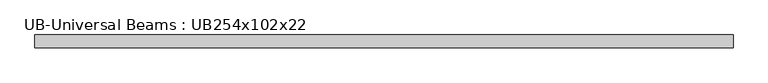
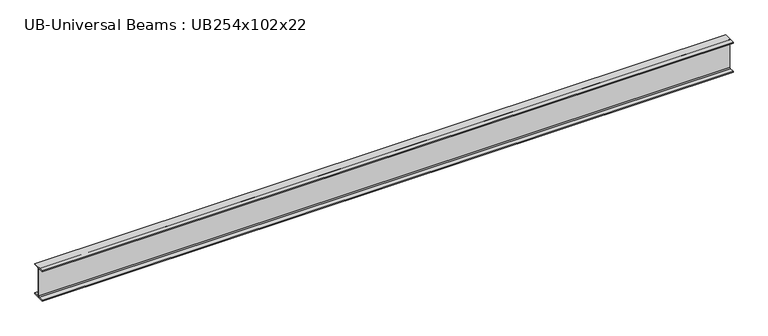
"""IFC4 building model written with IfcOpenShell, lengths in millimetres: beam geometry, UB-Universal Beams : UB254x102x22."""

import ifcopenshell
import ifcopenshell.guid

model = None  # the IFC model being written
_history = None  # IfcOwnerHistory: only IFC2X3 demands one
_inside = {}  # id of a spatial element -> (the spatial element, [elements in it])
_under = {}  # id of a project, library or spatial element -> (it, [spatial elements below it])
_declared = {}  # id of a project -> (the project, [libraries it declares])
_typed = {}  # id of a type object -> (the type object, [elements of that type])
_made_of = {}  # id of a material, layer set ... -> (it, [elements and type objects made of it])


def new_model(schema):
    """Start an empty IFC model of exactly this schema.

    Asked for "IFC4X3", IfcOpenShell would pick the latest addendum, in which some entities
    have other attributes; the version numbers below select the first issue.
    IFC2X3 requires an IfcOwnerHistory on every rooted entity: one is made here for all.
    """
    global model, _history
    if schema == "IFC4X3":
        model = ifcopenshell.file(schema_version=(4, 3, 0, 0))
    else:
        model = ifcopenshell.file(schema=schema)
    _inside.clear()
    _under.clear()
    _declared.clear()
    _typed.clear()
    _made_of.clear()
    _history = None
    if model.schema == "IFC2X3":
        org = make("IfcOrganization", Name="unknown")
        user = make(
            "IfcPersonAndOrganization",
            ThePerson=make("IfcPerson", FamilyName="unknown"),
            TheOrganization=org,
        )
        app = make(
            "IfcApplication",
            ApplicationDeveloper=org,
            Version="unknown",
            ApplicationFullName="unknown",
            ApplicationIdentifier="unknown",
        )
        _history = make(
            "IfcOwnerHistory",
            OwningUser=user,
            OwningApplication=app,
            ChangeAction="ADDED",
            CreationDate=0,
        )
    return model


def make(cls, **values):
    """One entity of the class cls with the attributes given. An attribute that is None is left unset."""
    return model.create_entity(
        cls, **{name: value for name, value in values.items() if value is not None}
    )


def rooted(cls, **values):
    """An entity with a GlobalId (a new one), such as an element, a storey or a relation."""
    return make(cls, GlobalId=ifcopenshell.guid.new(), OwnerHistory=_history, **values)


def si_unit(unit_type, name, prefix=None):
    """IfcSIUnit, for example si_unit("LENGTHUNIT", "METRE", prefix="MILLI")."""
    return make("IfcSIUnit", UnitType=unit_type, Prefix=prefix, Name=name)


def assignment(units):
    """IfcUnitAssignment: the units of a project."""
    return None if units is None else make("IfcUnitAssignment", Units=units)


def point(xyz):
    """IfcCartesianPoint."""
    return None if xyz is None else make("IfcCartesianPoint", Coordinates=xyz)


def direction(xyz):
    """IfcDirection."""
    return None if xyz is None else make("IfcDirection", DirectionRatios=xyz)


def frame(location, z_axis=None, x_axis=None):
    """IfcAxis2Placement3D, a coordinate frame: its origin and axes. An axis left out is left unset."""
    return make(
        "IfcAxis2Placement3D",
        Location=point(location),
        Axis=direction(z_axis),
        RefDirection=direction(x_axis),
    )


def frame_2d(location, x_axis=None):
    """IfcAxis2Placement2D, a coordinate frame in the plane: its origin and x axis."""
    return make(
        "IfcAxis2Placement2D", Location=point(location), RefDirection=direction(x_axis)
    )


def origin():
    """The frame at (0, 0, 0) with its axes left unset."""
    return frame((0.0, 0.0, 0.0))


def place(relative_to, where):
    """IfcLocalPlacement: puts the frame where relative to a parent placement (None: the world)."""
    return make(
        "IfcLocalPlacement", PlacementRelTo=relative_to, RelativePlacement=where
    )


def context(
    kind, dimensions, precision=None, world=None, true_north=None, identifier=None
):
    """IfcGeometricRepresentationContext, for example the 3D "Model" context."""
    return make(
        "IfcGeometricRepresentationContext",
        ContextIdentifier=identifier,
        ContextType=kind,
        CoordinateSpaceDimension=dimensions,
        Precision=precision,
        WorldCoordinateSystem=world,
        TrueNorth=true_north,
    )


def project(units=None, contexts=None):
    """IfcProject with its units and contexts."""
    return rooted(
        "IfcProject",
        Name="project",
        RepresentationContexts=contexts,
        UnitsInContext=assignment(units),
    )


def spatial(cls, under=None, at=None, **own):
    """A site, building, storey or space (cls), placed at a placement, below another one or the project."""
    s = rooted(cls, ObjectPlacement=at, **own)
    if under is not None:
        _under.setdefault(under.id(), (under, []))[1].append(s)
    return s


def polyline(points):
    """IfcPolyline through the points."""
    return make("IfcPolyline", Points=[point(p) for p in points])


def circle_curve(where, radius):
    """IfcCircle in the frame where."""
    return make("IfcCircle", Position=where, Radius=radius)


def trimmed(basis, trim1, trim2, sense, master):
    """IfcTrimmedCurve: the piece of a basis curve between two trims."""
    return make(
        "IfcTrimmedCurve",
        BasisCurve=basis,
        Trim1=trim1,
        Trim2=trim2,
        SenseAgreement=sense,
        MasterRepresentation=master,
    )


def segment(curve, same_sense, transition):
    """IfcCompositeCurveSegment."""
    return make(
        "IfcCompositeCurveSegment",
        Transition=transition,
        SameSense=same_sense,
        ParentCurve=curve,
    )


def composite_curve(segments, self_intersect=None):
    """IfcCompositeCurve: segments joined end to end."""
    return make("IfcCompositeCurve", Segments=segments, SelfIntersect=self_intersect)


def outline(outer, holes=None, kind="AREA"):
    """IfcArbitraryClosedProfileDef: a profile drawn as a closed curve; with holes, ...WithVoids."""
    if holes is None:
        return make("IfcArbitraryClosedProfileDef", ProfileType=kind, OuterCurve=outer)
    return make(
        "IfcArbitraryProfileDefWithVoids",
        ProfileType=kind,
        OuterCurve=outer,
        InnerCurves=holes,
    )


def extrude(swept, where, along, depth):
    """IfcExtrudedAreaSolid: the profile swept, set in the frame where, extruded along a direction by depth."""
    return make(
        "IfcExtrudedAreaSolid",
        SweptArea=swept,
        Position=where,
        ExtrudedDirection=direction(along),
        Depth=depth,
    )


def shape(context_of_items, identifier, shape_type, items):
    """IfcShapeRepresentation: the items that make up one representation, for example the "Body"."""
    return make(
        "IfcShapeRepresentation",
        ContextOfItems=context_of_items,
        RepresentationIdentifier=identifier,
        RepresentationType=shape_type,
        Items=items,
    )


def source(mapping_origin, context_of_items, identifier, shape_type, items):
    """IfcRepresentationMap: a shape defined once, which mapped items show again and again."""
    return make(
        "IfcRepresentationMap",
        MappingOrigin=mapping_origin,
        MappedRepresentation=shape(context_of_items, identifier, shape_type, items),
    )


def transform(
    local_origin,
    x_axis=None,
    y_axis=None,
    z_axis=None,
    scale=None,
    scale2=None,
    scale3=None,
    uniform=True,
):
    """IfcCartesianTransformationOperator3D, or its non-uniform kind. x_axis, y_axis, z_axis: its Axis1, 2, 3."""
    if uniform:
        return make(
            "IfcCartesianTransformationOperator3D",
            Axis1=direction(x_axis),
            Axis2=direction(y_axis),
            LocalOrigin=point(local_origin),
            Scale=scale,
            Axis3=direction(z_axis),
        )
    return make(
        "IfcCartesianTransformationOperator3DnonUniform",
        Axis1=direction(x_axis),
        Axis2=direction(y_axis),
        LocalOrigin=point(local_origin),
        Scale=scale,
        Axis3=direction(z_axis),
        Scale2=scale2,
        Scale3=scale3,
    )


def mapped(mapping_source, mapping_target):
    """IfcMappedItem: shows the shape of a source again, moved by a transform."""
    return make(
        "IfcMappedItem", MappingSource=mapping_source, MappingTarget=mapping_target
    )


def made_of(thing, what):
    """Note that an element or type object is made of a material, layer set ...; save() writes the relation."""
    if what is not None:
        _made_of.setdefault(what.id(), (what, []))[1].append(thing)
    return thing


def element(
    cls,
    number,
    at=None,
    inside=None,
    cuts=None,
    type_object=None,
    material=None,
    context=None,
    identifier="Body",
    shape_type=None,
    held_by="IfcProductDefinitionShape",
    body=None,
    shapes=None,
    **own,
):
    """One element of the class cls, such as IfcWall. Its Tag is "e" and its number.

    at: its placement. inside: the storey or other place that contains it. cuts: it is an
    opening in that element (IfcRelVoidsElement). A single representation is given by context,
    identifier, shape_type and body (its items); several are given by shapes. held_by: the class
    of the entity that holds the representations. save() writes the other relations.
    """
    e = rooted(cls, Tag="e%d" % number, ObjectPlacement=at, **own)
    if body is not None:
        shapes = [shape(context, identifier, shape_type, body)]
    if shapes is not None:
        e.Representation = make(held_by, Representations=shapes)
    if inside is not None:
        _inside.setdefault(inside.id(), (inside, []))[1].append(e)
    if cuts is not None:
        rooted(
            "IfcRelVoidsElement", RelatingBuildingElement=cuts, RelatedOpeningElement=e
        )
    if type_object is not None:
        _typed.setdefault(type_object.id(), (type_object, []))[1].append(e)
    return made_of(e, material)


def aggregate(whole, parts):
    """IfcRelAggregates: a whole, such as a stair, and the parts it consists of."""
    return rooted("IfcRelAggregates", RelatingObject=whole, RelatedObjects=parts)


def save(model, path):
    """Write the relations noted so far, then the file.

    IfcRelAggregates (storeys below a building ...), IfcRelContainedInSpatialStructure (elements
    in a storey), IfcRelDefinesByType, IfcRelAssociatesMaterial and IfcRelDeclares: one each for
    every whole, place, type object, material and project.
    """
    for whole, parts in _under.values():
        aggregate(whole, parts)
    for where, things in _inside.values():
        rooted(
            "IfcRelContainedInSpatialStructure",
            RelatedElements=things,
            RelatingStructure=where,
        )
    for kind, things in _typed.values():
        rooted("IfcRelDefinesByType", RelatedObjects=things, RelatingType=kind)
    for what, things in _made_of.values():
        rooted("IfcRelAssociatesMaterial", RelatedObjects=things, RelatingMaterial=what)
    for by, libraries in _declared.values():
        rooted("IfcRelDeclares", RelatingContext=by, RelatedDefinitions=libraries)
    model.write(path)


def ub_universal_beams_ub254x102x22_9642d6a0(model_context):
    return source(origin(), model_context, "Body", "SweptSolid", [
        extrude(outline(composite_curve([segment(polyline([(50.8, -120.2), (50.8, -127.0), (-50.8, -127.0), (-50.8, -120.2), (-10.45, -120.2)]), True, "CONTINUOUS"), segment(trimmed(circle_curve(frame_2d((-10.45, -112.6)), 7.6), [point((-10.45, -120.2))], [point((-2.85, -112.6))], True, "CARTESIAN"), True, "CONTINUOUS"), segment(polyline([(-2.85, -112.6), (-2.85, 112.6)]), True, "CONTINUOUS"), segment(trimmed(circle_curve(frame_2d((-10.45, 112.6)), 7.6), [point((-2.85, 112.6))], [point((-10.45, 120.2))], True, "CARTESIAN"), True, "CONTINUOUS"), segment(polyline([(-10.45, 120.2), (-50.8, 120.2), (-50.8, 127.0), (50.8, 127.0), (50.8, 120.2), (10.45, 120.2)]), True, "CONTINUOUS"), segment(trimmed(circle_curve(frame_2d((10.45, 112.6)), 7.6), [point((10.45, 120.2))], [point((2.85, 112.6))], True, "CARTESIAN"), True, "CONTINUOUS"), segment(polyline([(2.85, 112.6), (2.85, -112.6)]), True, "CONTINUOUS"), segment(trimmed(circle_curve(frame_2d((10.45, -112.6)), 7.6), [point((2.85, -112.6))], [point((10.45, -120.2))], True, "CARTESIAN"), True, "CONTINUOUS"), segment(polyline([(10.45, -120.2), (50.8, -120.2)]), True, "CONTINUOUS")], self_intersect=False)), frame((-2762.4, 0.0, 0.0), z_axis=(1.0, 0.0, 0.0), x_axis=(0.0, 1.0, 0.0)), (0.0, 0.0, 1.0), 5524.8),
    ])


if __name__ == "__main__":
    model = new_model("IFC4")
    model_context = context("Model", 3, world=origin())
    ifc_project = project(units=[si_unit("LENGTHUNIT", "METRE", prefix="MILLI")], contexts=[model_context])
    site = spatial("IfcSite", under=ifc_project)
    building = spatial("IfcBuilding", under=site)
    placement = place(None, origin())
    ub_universal_beams_ub254x102x22_shape = ub_universal_beams_ub254x102x22_9642d6a0(model_context)
    element("IfcBeam", 1, ObjectType="UB-Universal Beams : UB254x102x22", at=placement, inside=building, context=model_context, shape_type="MappedRepresentation", body=[
        mapped(ub_universal_beams_ub254x102x22_shape, transform((0.0, 0.0, 0.0), x_axis=(1.0, 0.0, 0.0), y_axis=(0.0, 1.0, 0.0), z_axis=(0.0, 0.0, 1.0))),
    ])
    save(model, "model.ifc")

# Revit data of these elements
# Type "UB-Universal Beams : UB254x102x22"
#   Section Name Key = "UB254X102X22"
#   Width = 10.16 cm
#   Web Thickness = 0.57 cm
#   Web Fillet = 0.76 cm
#   Warping Constant = 18200.0 cm⁶
#   Torsional Moment of Inertia = 4.15 cm⁴
#   Section Area = 28.0 cm²
#   Plastic Modulus weak axis = 37.3 cm³
#   Plastic Modulus strong axis = 259.0 cm³
#   Nominal Weight = 22.00 kgf/m
#   Moment of Inertia weak axis = 119.00 cm⁴
#   Moment of Inertia strong axis = 2841.00 cm⁴
#   Height = 25.4 cm
#   Flange Thickness = 0.68 cm
#   Elastic Modulus weak axis = 23.5 cm³
#   Elastic Modulus strong axis = 224.0 cm³
#   Centroid Vertical = 12.7 cm
#   Centroid Horizontal = 5.08 cm
#   Bolt Spacing = 5.4 cm
#   Length [instance default] = 1500 mm
#   Structural Material [instance default] = Metal - Steel 43-275
#   Type Comments = ""
#   Assembly Code = ""
# Element 1 (IfcBeam, "UB-Universal Beams : UB254x102x22")
#   Materials on its faces: "Metal - Steel 43-275"
# Materials
#   "Metal - Steel 43-275": class "Metal", colour RGB 247 247 247, transparency 0, Cost = 0
